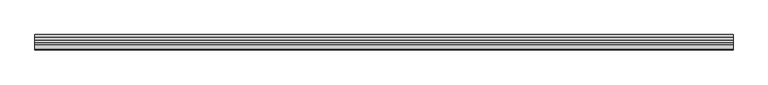
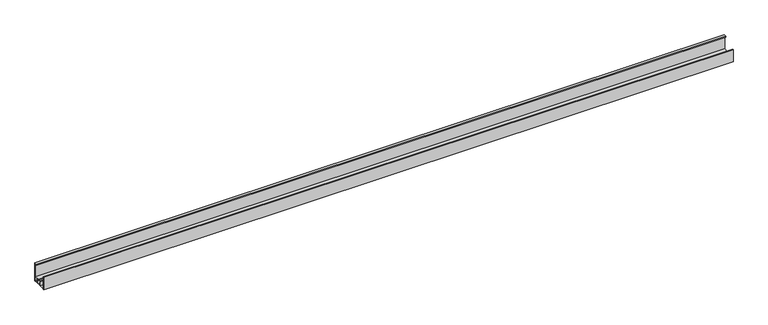
"""IFC4 building model written with IfcOpenShell, lengths in millimetres: proxy geometry, Generic Models 3:Generic Models 2:312240:Generic Models 2:312240 : Generic Models 3:Generic Models 2:312240:1 : Generic Models 3:Generic Models 2:312240:Generic Models 2:312240 : Generic Models 3:Generic Models 2:312240:300533."""

from ifc_helpers import new_model, si_unit, frame, origin, place, context, project, spatial, polyline, outline, extrude, source, transform, mapped, element, save


def generic_models_6e54990c(model_context):
    return source(origin(), model_context, "Body", "SweptSolid", [
        extrude(outline(polyline([(-579064.435512, 21.6981223), (-579047.8832558, 21.6981223), (-579047.8832558, 17.0006236), (-579049.8086712, 17.0006236), (-579049.8086712, 14.6193736), (-579047.8832558, 14.6193736), (-579047.8832558, 9.921875), (-579064.435512, 9.921875), (-579064.435512, 14.6193736), (-579062.5100965, 14.6193736), (-579062.5100965, 17.0006236), (-579064.435512, 17.0006236), (-579064.435512, 21.6981223)])), frame((590317.0242239, 0.0, 0.0), z_axis=(1.0, 0.0, 0.0), x_axis=(0.0, 1.0, 0.0)), (0.0, 0.0, 1.0), 2438.4),
        extrude(outline(polyline([(-579040.8458673, 74.35), (-579032.3994958, 74.35), (-579032.3994958, 6.35), (-579033.9869958, 6.35), (-579033.9869958, 7.9375), (-579051.6535683, 7.9375), (-579051.6535683, 9.525), (-579047.4863808, 9.525), (-579047.4863808, 15.0162486), (-579049.4117962, 15.0162486), (-579049.4117962, 16.6037486), (-579047.4863808, 16.6037486), (-579047.4863808, 22.0949973), (-579051.6535683, 22.0949973), (-579051.6535683, 23.6824973), (-579033.9869958, 23.6824973), (-579033.9869958, 72.7625), (-579039.2583673, 72.7625), (-579039.2583673, 69.9626734), (-579040.8458673, 69.9626734), (-579040.8458673, 74.35)]), holes=[polyline([(-579033.9869958, 22.0949973), (-579045.8988808, 22.0949973), (-579045.8988808, 9.525), (-579033.9869958, 9.525), (-579033.9869958, 22.0949973)])]), frame((590317.0242239, 0.0, 0.0), z_axis=(1.0, 0.0, 0.0), x_axis=(0.0, 1.0, 0.0)), (0.0, 0.0, 1.0), 2438.4),
        extrude(outline(polyline([(-579084.8119958, 6.35), (-579086.3994958, 6.35), (-579086.3994958, 52.3546875), (-579083.6844059, 52.3546875), (-579083.6844059, 50.7671875), (-579084.8119958, 50.7671875), (-579084.8119958, 9.525), (-579066.419887, 9.525), (-579066.419887, 23.6824973), (-579060.6651995, 23.6824973), (-579060.6651995, 22.0949973), (-579064.832387, 22.0949973), (-579064.832387, 16.6037486), (-579062.9069715, 16.6037486), (-579062.9069715, 15.0162486), (-579064.832387, 15.0162486), (-579064.832387, 9.525), (-579060.6651995, 9.525), (-579060.6651995, 7.9375), (-579084.8119958, 7.9375), (-579084.8119958, 6.35)])), frame((590317.0242239, 0.0, 0.0), z_axis=(1.0, 0.0, 0.0), x_axis=(0.0, 1.0, 0.0)), (0.0, 0.0, 1.0), 2438.4),
    ])


if __name__ == "__main__":
    model = new_model("IFC4")
    model_context = context("Model", 3, world=origin())
    ifc_project = project(units=[si_unit("LENGTHUNIT", "METRE", prefix="MILLI")], contexts=[model_context])
    site = spatial("IfcSite", under=ifc_project)
    building = spatial("IfcBuilding", under=site)
    placement = place(None, origin())
    generic_models_shape = generic_models_6e54990c(model_context)
    element("IfcBuildingElementProxy", 1, Name="Generic Models 3:Generic Models 2:312240:Generic Models 2:312240 : Generic Models 3:Generic Models 2:312240:1 : Generic Models 3:Generic Models 2:312240:Generic Models 2:312240 : Generic Models 3:Generic Models 2:312240:300533", ObjectType="Generic Models 3:Generic Models 2:312240:Generic Models 2:312240 : Generic Models 3:Generic Models 2:312240:1 : Generic Models 3:Generic Models 2:312240:Generic Models 2:312240 : Generic Models 3:Generic Models 2:312240:300533", at=placement, inside=building, context=model_context, shape_type="MappedRepresentation", body=[
        mapped(generic_models_shape, transform((0.0, 0.0, 0.0), x_axis=(1.0, 0.0, 0.0), y_axis=(0.0, 1.0, 0.0), z_axis=(0.0, 0.0, 1.0))),
    ])
    save(model, "model.ifc")

# Revit data of these elements
# Type "Generic Models 3:Generic Models 2:312240:Generic Models 2:312240 : Generic Models 3:Generic Models 2:312240:1 : Generic Models 3:Generic Models 2:312240:Generic Models 2:312240 : Generic Models 3:Generic Models 2:312240:300533"
#   NameOverride = "Generic Models 3:Generic Models 2:312240:Generic Models 2:312240 : Generic Models 3:Generic Models 2:312240:300533"
#   ObjectTypeOverride = "Generic Models 2:312240 : Generic Models 3:Generic Models 2:312240"
#   Reference = "Generic Models 2"
#   Tag = "300533"
# Element 1 (IfcBuildingElementProxy, "Generic Models 3:Generic Models 2:312240:Generic Models 2:312240 : Generic Models 3:Generic Models 2:312240:1 : Generic Models 3:Generic Models 2:312240:Generic Models 2:312240 : Generic Models 3:Generic Models 2:312240:300533")
#   Materials on its faces: "THERMAL BROKEN ALUMINUM STOREFRONT FOR POLYCARBONATE"
# Materials
#   "THERMAL BROKEN ALUMINUM STOREFRONT FOR POLYCARBONATE": class "Unassigned", colour RGB 244 244 244, transparency 0, Keynote = "M07611300.01", Cost = 0
